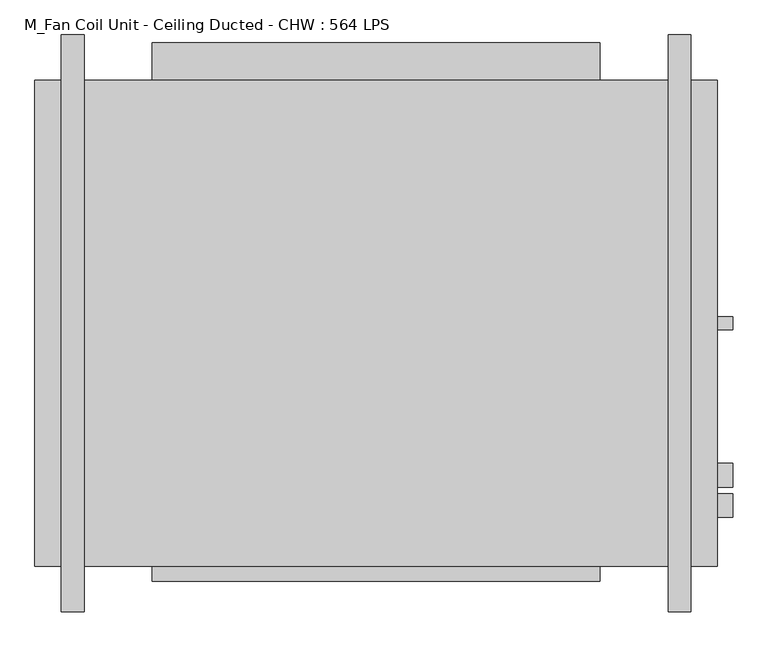
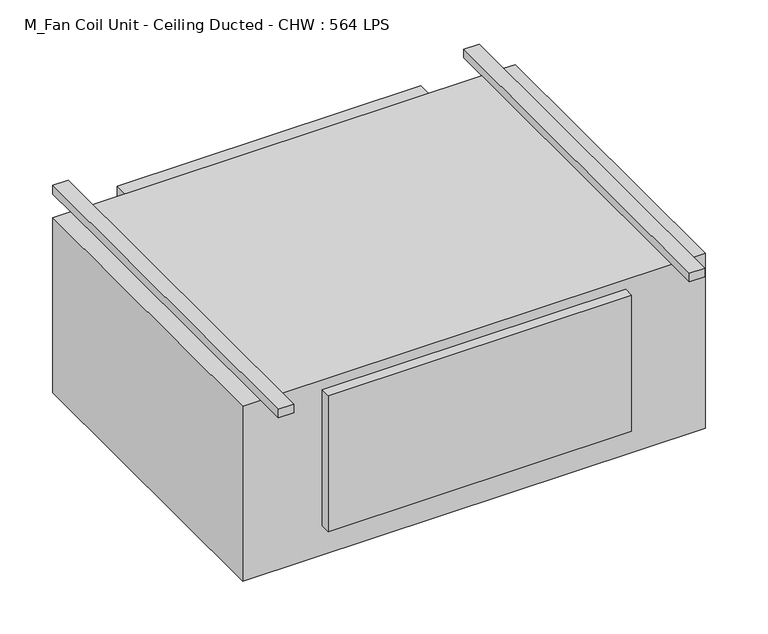
"""IFC4 building model written with IfcOpenShell, lengths in millimetres: proxy geometry, M_Fan Coil Unit - Ceiling Ducted - CHW : 564 LPS."""

from ifc_helpers import new_model, si_unit, frame, origin, place, context, project, spatial, circle_curve, source, transform, mapped, element, save
from ifc_brep_helpers import plane_surface, cylinder_surface, advanced_brep


def m_fan_coil_unit_ceiling_ducted_chw_564_lps_c1f53b58(model_context):
    return source(origin(), model_context, "Body", "AdvancedBrep", [
        advanced_brep(
        [(82.55, 889.0, 479.425), (44.45, 889.0, 479.425), (44.45, -76.2, 479.425), (82.55, -76.2, 479.425), (82.55, -76.2, 457.2), (44.45, -76.2, 457.2), (44.45, 0.0, 457.2), (82.55, 0.0, 457.2), (44.45, 889.0, 457.2), (82.55, 889.0, 457.2), (82.55, 812.8, 457.2), (44.45, 812.8, 457.2), (1098.55, 889.0, 479.425), (1060.45, 889.0, 479.425), (1060.45, -76.2, 479.425), (1098.55, -76.2, 479.425), (1098.55, -76.2, 457.2), (1060.45, -76.2, 457.2), (1060.45, 0.0, 457.2), (1098.55, 0.0, 457.2), (1060.45, 889.0, 457.2), (1098.55, 889.0, 457.2), (1098.55, 812.8, 457.2), (1060.45, 812.8, 457.2), (1168.4, 132.4, 381.0), (1168.4, 172.4, 381.0), (1143.0, 132.4, 381.0), (1143.0, 172.4, 381.0), (1168.4, 81.6, 101.6), (1168.4, 121.6, 101.6), (1143.0, 81.6, 101.6), (1143.0, 121.6, 101.6), (1168.4, 395.2875, 38.1), (1168.4, 417.5125, 38.1), (1143.0, 395.2875, 38.1), (1143.0, 417.5125, 38.1), (0.0, 812.8, 457.2), (0.0, 0.0, 457.2), (1143.0, 0.0, 457.2), (1143.0, 812.8, 457.2), (1143.0, 812.8, 0.0), (1143.0, 0.0, 0.0), (0.0, 0.0, 0.0), (0.0, 812.8, 0.0), (946.5, 812.8, 431.8), (196.5, 812.8, 431.8), (196.5, 812.8, 76.2), (946.5, 812.8, 76.2), (196.5, 0.0, 431.8), (946.5, 0.0, 431.8), (946.5, 0.0, 76.2), (196.5, 0.0, 76.2), (946.5, 876.3, 431.8), (196.5, 876.3, 431.8), (946.5, 876.3, 76.2), (196.5, 876.3, 76.2), (196.5, -25.4, 431.8), (946.5, -25.4, 431.8), (946.5, -25.4, 76.2), (196.5, -25.4, 76.2)],
        [
            (0, 1),
            (1, 2),
            (2, 3),
            (3, 0),
            (4, 5),
            (5, 6),
            (6, 7),
            (7, 4),
            (8, 9),
            (9, 10),
            (10, 11),
            (11, 8),
            (0, 9),
            (8, 1),
            (11, 6),
            (5, 2),
            (4, 3),
            (7, 10),
            (12, 13),
            (13, 14),
            (14, 15),
            (15, 12),
            (16, 17),
            (17, 18),
            (18, 19),
            (19, 16),
            (20, 21),
            (21, 22),
            (22, 23),
            (23, 20),
            (12, 21),
            (20, 13),
            (23, 18),
            (17, 14),
            (16, 15),
            (19, 22),
            (24, 25, circle_curve(frame((1168.4, 152.4, 381.0), z_axis=(1.0, 0.0, 0.0), x_axis=(0.0, 1.0, 0.0)), 20.0)),
            (25, 24, circle_curve(frame((1168.4, 152.4, 381.0), z_axis=(1.0, 0.0, 0.0), x_axis=(0.0, 1.0, 0.0)), 20.0)),
            (24, 26),
            (26, 27, circle_curve(frame((1143.0, 152.4, 381.0), z_axis=(1.0, 0.0, 0.0), x_axis=(0.0, 1.0, 0.0)), 20.0)),
            (27, 25),
            (27, 26, circle_curve(frame((1143.0, 152.4, 381.0), z_axis=(1.0, 0.0, 0.0), x_axis=(0.0, 1.0, 0.0)), 20.0)),
            (28, 29, circle_curve(frame((1168.4, 101.6, 101.6), z_axis=(1.0, 0.0, 0.0), x_axis=(0.0, 1.0, 0.0)), 20.0)),
            (29, 28, circle_curve(frame((1168.4, 101.6, 101.6), z_axis=(1.0, 0.0, 0.0), x_axis=(0.0, 1.0, 0.0)), 20.0)),
            (28, 30),
            (30, 31, circle_curve(frame((1143.0, 101.6, 101.6), z_axis=(1.0, 0.0, 0.0), x_axis=(0.0, 1.0, 0.0)), 20.0)),
            (31, 29),
            (31, 30, circle_curve(frame((1143.0, 101.6, 101.6), z_axis=(1.0, 0.0, 0.0), x_axis=(0.0, 1.0, 0.0)), 20.0)),
            (32, 33, circle_curve(frame((1168.4, 406.4, 38.1), z_axis=(1.0, 0.0, 0.0), x_axis=(0.0, 1.0, 0.0)), 11.1125)),
            (33, 32, circle_curve(frame((1168.4, 406.4, 38.1), z_axis=(1.0, 0.0, 0.0), x_axis=(0.0, 1.0, 0.0)), 11.1125)),
            (32, 34),
            (34, 35, circle_curve(frame((1143.0, 406.4, 38.1), z_axis=(1.0, 0.0, 0.0), x_axis=(0.0, 1.0, 0.0)), 11.1125)),
            (35, 33),
            (35, 34, circle_curve(frame((1143.0, 406.4, 38.1), z_axis=(1.0, 0.0, 0.0), x_axis=(0.0, 1.0, 0.0)), 11.1125)),
            (36, 37),
            (37, 6),
            (11, 36),
            (38, 39),
            (39, 22),
            (19, 38),
            (23, 10),
            (7, 18),
            (40, 41),
            (41, 42),
            (42, 43),
            (43, 40),
            (43, 36),
            (39, 40),
            (44, 45),
            (45, 46),
            (46, 47),
            (47, 44),
            (42, 37),
            (41, 38),
            (48, 49),
            (49, 50),
            (50, 51),
            (51, 48),
            (52, 53),
            (53, 45),
            (44, 52),
            (54, 47),
            (46, 55),
            (55, 54),
            (52, 54),
            (55, 53),
            (48, 56),
            (56, 57),
            (57, 49),
            (50, 58),
            (58, 59),
            (59, 51),
            (59, 56),
            (58, 57),
        ],
        [
            plane_surface(frame((44.45, 889.0, 479.425), z_axis=(0.0, 0.0, 1.0), x_axis=(-1.0, 0.0, 0.0))),
            plane_surface(frame((44.45, 889.0, 457.2), z_axis=(0.0, 0.0, -1.0), x_axis=(1.0, 0.0, 0.0))),
            plane_surface(frame((82.55, 889.0, 479.425), z_axis=(0.0, 1.0, 0.0), x_axis=(0.0, 0.0, -1.0))),
            plane_surface(frame((44.45, 889.0, 479.425), z_axis=(-1.0, 0.0, 0.0), x_axis=(0.0, 0.0, -1.0))),
            plane_surface(frame((44.45, -76.2, 479.425), z_axis=(0.0, -1.0, 0.0), x_axis=(0.0, 0.0, -1.0))),
            plane_surface(frame((82.55, -76.2, 479.425), z_axis=(1.0, 0.0, 0.0), x_axis=(0.0, 0.0, -1.0))),
            plane_surface(frame((1060.45, 889.0, 479.425), z_axis=(0.0, 0.0, 1.0), x_axis=(-1.0, 0.0, 0.0))),
            plane_surface(frame((1060.45, 889.0, 457.2), z_axis=(0.0, 0.0, -1.0), x_axis=(1.0, 0.0, 0.0))),
            plane_surface(frame((1098.55, 889.0, 479.425), z_axis=(0.0, 1.0, 0.0), x_axis=(0.0, 0.0, -1.0))),
            plane_surface(frame((1060.45, 889.0, 479.425), z_axis=(-1.0, 0.0, 0.0), x_axis=(0.0, 0.0, -1.0))),
            plane_surface(frame((1060.45, -76.2, 479.425), z_axis=(0.0, -1.0, 0.0), x_axis=(0.0, 0.0, -1.0))),
            plane_surface(frame((1098.55, -76.2, 479.425), z_axis=(1.0, 0.0, 0.0), x_axis=(0.0, 0.0, -1.0))),
            plane_surface(frame((1168.4, 172.4, 381.0), z_axis=(1.0, 0.0, 0.0), x_axis=(0.0, 0.0, 1.0))),
            cylinder_surface(frame((1143.0, 152.4, 381.0), z_axis=(1.0, 0.0, 0.0), x_axis=(0.0, 1.0, 0.0)), 20.0),
            plane_surface(frame((1168.4, 121.6, 101.6), z_axis=(1.0, 0.0, 0.0), x_axis=(0.0, 0.0, 1.0))),
            cylinder_surface(frame((1143.0, 101.6, 101.6), z_axis=(1.0, 0.0, 0.0), x_axis=(0.0, 1.0, 0.0)), 20.0),
            plane_surface(frame((1168.4, 417.5125, 38.1), z_axis=(1.0, 0.0, 0.0), x_axis=(0.0, 0.0, 1.0))),
            cylinder_surface(frame((1143.0, 406.4, 38.1), z_axis=(1.0, 0.0, 0.0), x_axis=(0.0, 1.0, 0.0)), 11.1125),
            plane_surface(frame((0.0, 812.8, 457.2), z_axis=(0.0, 0.0, 1.0), x_axis=(-1.0, 0.0, 0.0))),
            plane_surface(frame((0.0, 812.8, 0.0), z_axis=(0.0, 0.0, -1.0), x_axis=(1.0, 0.0, 0.0))),
            plane_surface(frame((1143.0, 812.8, 457.2), z_axis=(0.0, 1.0, 0.0), x_axis=(0.0, 0.0, -1.0))),
            plane_surface(frame((0.0, 812.8, 457.2), z_axis=(-1.0, 0.0, 0.0), x_axis=(0.0, 0.0, -1.0))),
            plane_surface(frame((0.0, 0.0, 457.2), z_axis=(0.0, -1.0, 0.0), x_axis=(0.0, 0.0, -1.0))),
            plane_surface(frame((1143.0, 0.0, 457.2), z_axis=(1.0, 0.0, 0.0), x_axis=(0.0, 0.0, -1.0))),
            plane_surface(frame((196.5, 876.3, 431.8), z_axis=(0.0, 0.0, 1.0), x_axis=(-1.0, 0.0, 0.0))),
            plane_surface(frame((196.5, 876.3, 76.2), z_axis=(0.0, 0.0, -1.0), x_axis=(1.0, 0.0, 0.0))),
            plane_surface(frame((946.5, 876.3, 431.8), z_axis=(0.0, 1.0, 0.0), x_axis=(0.0, 0.0, -1.0))),
            plane_surface(frame((196.5, 876.3, 431.8), z_axis=(-1.0, 0.0, 0.0), x_axis=(0.0, 0.0, -1.0))),
            plane_surface(frame((946.5, 812.8, 431.8), z_axis=(1.0, 0.0, 0.0), x_axis=(0.0, 0.0, -1.0))),
            plane_surface(frame((196.5, 0.0, 431.8), z_axis=(0.0, 0.0, 1.0), x_axis=(-1.0, 0.0, 0.0))),
            plane_surface(frame((196.5, 0.0, 76.2), z_axis=(0.0, 0.0, -1.0), x_axis=(1.0, 0.0, 0.0))),
            plane_surface(frame((196.5, 0.0, 431.8), z_axis=(-1.0, 0.0, 0.0), x_axis=(0.0, 0.0, -1.0))),
            plane_surface(frame((196.5, -25.4, 431.8), z_axis=(0.0, -1.0, 0.0), x_axis=(0.0, 0.0, -1.0))),
            plane_surface(frame((946.5, -25.4, 431.8), z_axis=(1.0, 0.0, 0.0), x_axis=(0.0, 0.0, -1.0))),
        ],
        [
            (0, [[1, 2, 3, 4]]),
            (1, [[5, 6, 7, 8]]),
            (1, [[9, 10, 11, 12]]),
            (2, [[-1, 13, -9, 14]]),
            (3, [[-2, -14, -12, 15, -6, 16]]),
            (4, [[-3, -16, -5, 17]]),
            (5, [[-4, -17, -8, 18, -10, -13]]),
            (6, [[19, 20, 21, 22]]),
            (7, [[23, 24, 25, 26]]),
            (7, [[27, 28, 29, 30]]),
            (8, [[-19, 31, -27, 32]]),
            (9, [[-20, -32, -30, 33, -24, 34]]),
            (10, [[-21, -34, -23, 35]]),
            (11, [[-22, -35, -26, 36, -28, -31]]),
            (12, [[37, 38]]),
            (13, [[-37, 39, 40, 41]]),
            (13, [[-38, -41, 42, -39]]),
            (14, [[43, 44]]),
            (15, [[-43, 45, 46, 47]]),
            (15, [[-44, -47, 48, -45]]),
            (16, [[49, 50]]),
            (17, [[-49, 51, 52, 53]]),
            (17, [[-50, -53, 54, -51]]),
            (18, [[55, 56, -15, 57]]),
            (18, [[58, 59, -36, 60]]),
            (18, [[61, -18, 62, -33]]),
            (19, [[63, 64, 65, 66]]),
            (20, [[-66, 67, -57, -11, -61, -29, -59, 68], [69, 70, 71, 72]]),
            (21, [[-55, -67, -65, 73]]),
            (22, [[-64, 74, -60, -25, -62, -7, -56, -73], [75, 76, 77, 78]]),
            (23, [[-58, -74, -63, -68], [-40, -42], [-46, -48], [-52, -54]]),
            (24, [[79, 80, -69, 81]]),
            (25, [[82, -71, 83, 84]]),
            (26, [[-79, 85, -84, 86]]),
            (27, [[-80, -86, -83, -70]]),
            (28, [[-81, -72, -82, -85]]),
            (29, [[87, 88, 89, -75]]),
            (30, [[90, 91, 92, -77]]),
            (31, [[-87, -78, -92, 93]]),
            (32, [[-88, -93, -91, 94]]),
            (33, [[-89, -94, -90, -76]]),
        ],
    ),
    ])


if __name__ == "__main__":
    model = new_model("IFC4")
    model_context = context("Model", 3, world=origin())
    ifc_project = project(units=[si_unit("LENGTHUNIT", "METRE", prefix="MILLI")], contexts=[model_context])
    site = spatial("IfcSite", under=ifc_project)
    building = spatial("IfcBuilding", under=site)
    placement = place(None, origin())
    m_fan_coil_unit_ceiling_ducted_chw_564_lps_shape = m_fan_coil_unit_ceiling_ducted_chw_564_lps_c1f53b58(model_context)
    element("IfcBuildingElementProxy", 1, Name="M_Fan Coil Unit - Ceiling Ducted - CHW : 564 LPS", ObjectType="M_Fan Coil Unit - Ceiling Ducted - CHW : 564 LPS", at=placement, inside=building, context=model_context, shape_type="MappedRepresentation", body=[
        mapped(m_fan_coil_unit_ceiling_ducted_chw_564_lps_shape, transform((0.0, 0.0, 0.0), x_axis=(1.0, 0.0, 0.0), y_axis=(0.0, 1.0, 0.0), z_axis=(0.0, 0.0, 1.0))),
    ])
    save(model, "model.ifc")

# Revit data of these elements
# Type "M_Fan Coil Unit - Ceiling Ducted - CHW : 564 LPS"
#   Water Pressure Drop [instance default] = 89631.8 Pa
#   Voltage = 120 V
#   Unit Length = 1143 mm
#   Total Cooling Capacity = 13950.2 W
#   Supply Water Radius = 20 mm
#   Supply Water Diameter = 40 mm
#   Supply Air Width = 750 mm
#   Sensible Cooling Capacity = 9466.2 W
#   Return Water Radius = 20 mm
#   Return Water Diameter = 40 mm
#   Return Air Width = 750 mm
#   Nominal Air Flow [instance default] = 566.34 L/s
#   External Static Pressure [instance default] = -74.65 Pa
#   Drain Flow [instance default] = 0.0 L/s
#   Chilled Water Flow [instance default] = 0.63 L/s
#   Apparent Load = 550 VA
#   Number of Poles = 1
#   Load Classification = Cooling
#   CFU Material = none
# Element 1 (IfcBuildingElementProxy, "M_Fan Coil Unit - Ceiling Ducted - CHW : 564 LPS")
#   Water Pressure Drop = 9652.66 Pa
#   Nominal Air Flow = 1175.0 L/s
#   External Static Pressure = 74.65 Pa
#   Chilled Water Flow = 0.25 L/s
